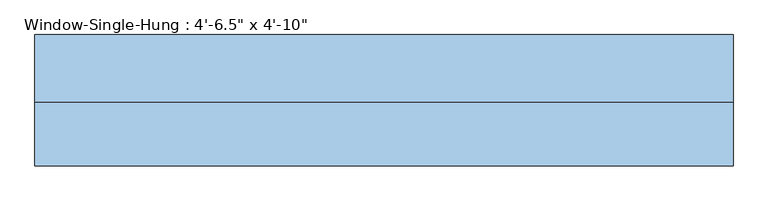
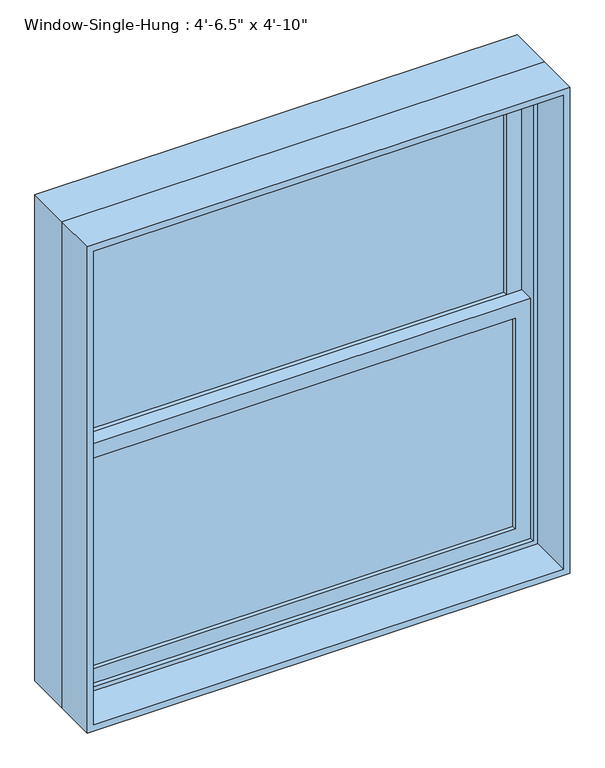
"""IFC4 building model written with IfcOpenShell, lengths in millimetres: window geometry."""

from ifc_helpers import new_model, si_unit, frame, origin, place, context, project, spatial, polyline, outline, extrude, source, transform, mapped, element, save


def window_bd35b4c6(model_context):
    return source(origin(), model_context, "Body", "SweptSolid", [
        extrude(outline(polyline([(615.95, 50.8), (615.95, 44.45), (-615.95, 44.45), (-615.95, 50.8), (615.95, 50.8)])), frame((0.0, 0.0, 990.6), z_axis=(0.0, 0.0, 1.0), x_axis=(1.0, 0.0, 0.0)), (0.0, 0.0, 1.0), 638.175),
        extrude(outline(polyline([(-615.95, 38.1), (615.95, 38.1), (615.95, 31.75), (-615.95, 31.75), (-615.95, 38.1)])), frame((0.0, 0.0, 990.6), z_axis=(0.0, 0.0, 1.0), x_axis=(1.0, 0.0, 0.0)), (0.0, 0.0, 1.0), 638.175),
        extrude(outline(polyline([(615.95, 95.25), (615.95, 88.9), (-615.95, 88.9), (-615.95, 95.25), (615.95, 95.25)])), frame((0.0, 0.0, 1673.225), z_axis=(0.0, 0.0, 1.0), x_axis=(1.0, 0.0, 0.0)), (0.0, 0.0, 1.0), 638.175),
        extrude(outline(polyline([(-615.95, 82.55), (615.95, 82.55), (615.95, 76.2), (-615.95, 76.2), (-615.95, 82.55)])), frame((0.0, 0.0, 1673.225), z_axis=(0.0, 0.0, 1.0), x_axis=(1.0, 0.0, 0.0)), (0.0, 0.0, 1.0), 638.175),
        extrude(outline(polyline([(1673.225, -660.4), (946.15, -660.4), (946.15, 660.4), (1673.225, 660.4), (1673.225, -660.4)]), holes=[polyline([(1628.775, 615.95), (990.6, 615.95), (990.6, -615.95), (1628.775, -615.95), (1628.775, 615.95)])]), frame((0.0, 19.05, 0.0), z_axis=(0.0, 1.0, 0.0), x_axis=(0.0, 0.0, 1.0)), (0.0, 0.0, 1.0), 44.45),
        extrude(outline(polyline([(2355.85, -660.4), (1628.775, -660.4), (1628.775, 660.4), (2355.85, 660.4), (2355.85, -660.4)]), holes=[polyline([(2311.4, 615.95), (1673.225, 615.95), (1673.225, -615.95), (2311.4, -615.95), (2311.4, 615.95)])]), frame((0.0, 63.5, 0.0), z_axis=(0.0, 1.0, 0.0), x_axis=(0.0, 0.0, 1.0)), (0.0, 0.0, 1.0), 44.45),
        extrude(outline(polyline([(2387.6, -692.15), (914.4, -692.15), (914.4, 692.15), (2387.6, 692.15), (2387.6, -692.15)]), holes=[polyline([(2355.85, 660.4), (946.15, 660.4), (946.15, -660.4), (2355.85, -660.4), (2355.85, 660.4)])]), frame((0.0, 6.35, 0.0), z_axis=(0.0, 1.0, 0.0), x_axis=(0.0, 0.0, 1.0)), (0.0, 0.0, 1.0), 133.35),
        extrude(outline(polyline([(2387.6, 692.15), (2387.6, -692.15), (914.4, -692.15), (914.4, 692.15), (2387.6, 692.15)]), holes=[polyline([(2368.55, 673.1), (933.45, 673.1), (933.45, -673.1), (2368.55, -673.1), (2368.55, 673.1)])]), frame((0.0, -120.65, 0.0), z_axis=(0.0, 1.0, 0.0), x_axis=(0.0, 0.0, 1.0)), (0.0, 0.0, 1.0), 127.0),
    ])


if __name__ == "__main__":
    model = new_model("IFC4")
    model_context = context("Model", 3, world=origin())
    ifc_project = project(units=[si_unit("LENGTHUNIT", "METRE", prefix="MILLI")], contexts=[model_context])
    site = spatial("IfcSite", under=ifc_project)
    building = spatial("IfcBuilding", under=site)
    placement = place(None, origin())
    window_shape = window_bd35b4c6(model_context)
    element("IfcWindow", 1, ObjectType="Window-Single-Hung : 4'-6.5\" x 4'-10\"", at=placement, inside=building, context=model_context, shape_type="MappedRepresentation", body=[
        mapped(window_shape, transform((0.0, 0.0, 0.0), x_axis=(1.0, 0.0, 0.0), y_axis=(0.0, 1.0, 0.0), z_axis=(0.0, 0.0, 1.0))),
    ])
    save(model, "model.ifc")

# Revit data of these elements
# Type "Window-Single-Hung : 4'-6.5\" x 4'-10\""
#   Type Mark = "10"
#   Fire Rating = "0.5h"
#   Construction Type Id = "DG-DR"
#   Assembly Code = "B2020100"
#   Analytic Construction = "Double glazing - domestic"
#   Wall Thickness [instance default] = 0' - 6"
#   Window Inset [instance default] = 0' - 0"
#   Visual Light Transmittance = 0.81
#   Thermal Resistance (R) = 0.319569 (m²·K)/W
#   Solar Heat Gain Coefficient = 0.76
#   Muntin Width = 4' - 0 1/2"
#   Muntin Height = 2' - 1 1/8"
#   Interior Wall Closure [instance default] = 0' - 1 1/2"
#   Rough Width = 4' - 7"
#   Rough Height = 4' - 10 1/2"
#   Frame Extension [instance default] = 0' - 1 1/4"
#   Exterior Wall Closure [instance default] = 0' - 0 1/2"
#   Extension Jamb [instance default] = 0' - 1 1/2"
#   Heat Transfer Coefficient (U) = 3.12929 W/(m²·K)
#   Height = 4' - 10"
#   Width = 4' - 6 1/2"
#   Top Muntin Visibility = no
#   Indicator Visibility = no
#   Extension Jamb Visibility [instance default] = yes
#   Interior Trim Visibility [instance default] = yes
#   Exterior Trim Visibility [instance default] = yes
#   Bottom Muntin Visibility = no
#   Muntin Pattern = Muntin Pattern_2x2 : Muntin Pattern_2x2
#   Interior Trim Material = 1X WOOD COMPOSITE TRIM
#   Interior Trim = Trim-Window-Interior-Flat : Picture Frame
#   Exterior Trim Material = 1X WOOD COMPOSITE TRIM
#   Exterior Trim = Trim-Window-Exterior-Flat : with Sill
#   Glass Panel Material = NEW DOUBLE HUNG WINDOWS (TYP.)
#   Exterior Frame Material = 1X WOOD COMPOSITE TRIM
#   Interior Frame Material = 1X WOOD COMPOSITE TRIM
#   Wall Closure = (empty or 0)
# Element 1 (IfcWindow, "Window-Single-Hung : 4'-6.5\" x 4'-10\"")
#   Wall Thickness = 0' - 9 1/2"
#   Extension Jamb = 0' - 5"
#   Materials on its faces: "1X WOOD COMPOSITE TRIM", "NEW DOUBLE HUNG WINDOWS (TYP.)"
# Materials
#   "1X WOOD COMPOSITE TRIM": class "Generic", colour RGB 88 61 61, transparency 0, Cost = 0
#   "NEW DOUBLE HUNG WINDOWS (TYP.)": class "Glass", colour RGB 218 227 224, transparency 0.85, Description = "Soda Lime Glass", Cost = 0
